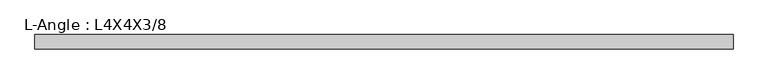
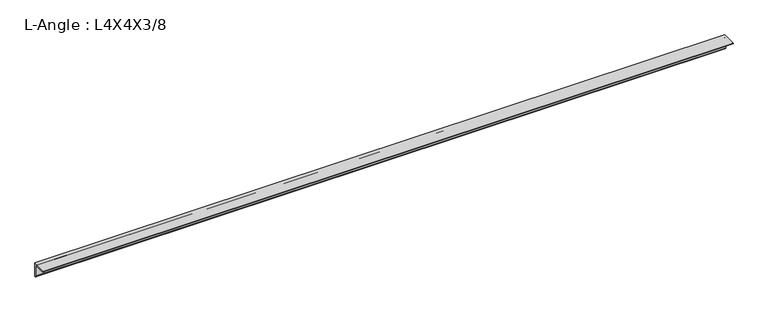
"""IFC4 building model written with IfcOpenShell, lengths in millimetres: beam geometry, L-Angle : L4X4X3/8."""

from ifc_helpers import new_model, si_unit, point, frame, frame_2d, origin, place, context, project, spatial, polyline, circle_curve, trimmed, segment, composite_curve, outline, extrude, source, transform, mapped, element, save


def l_angle_l4x4x3_8_aa974db8(model_context):
    return source(origin(), model_context, "Body", "SweptSolid", [
        extrude(outline(composite_curve([segment(polyline([(28.702, 28.702), (28.702, -72.898)]), True, "CONTINUOUS"), segment(trimmed(circle_curve(frame_2d((28.702, -63.373)), 9.525), [point((28.702, -72.898))], [point((19.177, -63.373))], False, "CARTESIAN"), True, "CONTINUOUS"), segment(polyline([(19.177, -63.373), (19.177, 9.652)]), True, "CONTINUOUS"), segment(trimmed(circle_curve(frame_2d((9.652, 9.652)), 9.525), [point((19.177, 9.652))], [point((9.652, 19.177))], True, "CARTESIAN"), True, "CONTINUOUS"), segment(polyline([(9.652, 19.177), (-63.373, 19.177)]), True, "CONTINUOUS"), segment(trimmed(circle_curve(frame_2d((-63.373, 28.702)), 9.525), [point((-63.373, 19.177))], [point((-72.898, 28.702))], False, "CARTESIAN"), True, "CONTINUOUS"), segment(polyline([(-72.898, 28.702), (28.702, 28.702)]), True, "CONTINUOUS")], self_intersect=False)), frame((-2476.5, 0.0, 0.0), z_axis=(1.0, 0.0, 0.0), x_axis=(0.0, 1.0, 0.0)), (0.0, 0.0, 1.0), 4864.1),
    ])


if __name__ == "__main__":
    model = new_model("IFC4")
    model_context = context("Model", 3, world=origin())
    ifc_project = project(units=[si_unit("LENGTHUNIT", "METRE", prefix="MILLI")], contexts=[model_context])
    site = spatial("IfcSite", under=ifc_project)
    building = spatial("IfcBuilding", under=site)
    placement = place(None, origin())
    l_angle_l4x4x3_8_shape = l_angle_l4x4x3_8_aa974db8(model_context)
    element("IfcBeam", 1, ObjectType="L-Angle : L4X4X3/8", at=placement, inside=building, context=model_context, shape_type="MappedRepresentation", body=[
        mapped(l_angle_l4x4x3_8_shape, transform((0.0, 0.0, 0.0), x_axis=(1.0, 0.0, 0.0), y_axis=(0.0, 1.0, 0.0), z_axis=(0.0, 0.0, 1.0))),
    ])
    save(model, "model.ifc")

# Revit data of these elements
# Type "L-Angle : L4X4X3/8"
#   Assembly Code = "B10"
#   k = 0' - 0 3/4"
#   W = 9.8
#   Length [instance default] = 5' - 0"
#   b = 0' - 4"
#   d = 0' - 4"
#   t = 0' - 0 3/8"
#   x = 0' - 1.13"
#   y = 0' - 1.13"
#   A = 0.0198611 SF
#   Structural Material [instance default] = Steel ASTM A36
# Element 1 (IfcBeam, "L-Angle : L4X4X3/8")
#   Materials on its faces: "Steel ASTM A36"
# Materials
#   "Steel ASTM A36": class "Metal", colour RGB 199 199 199, transparency 0, Description = "Structural steel, ASTM A36 Grade B, mill finish", Cost = 0
